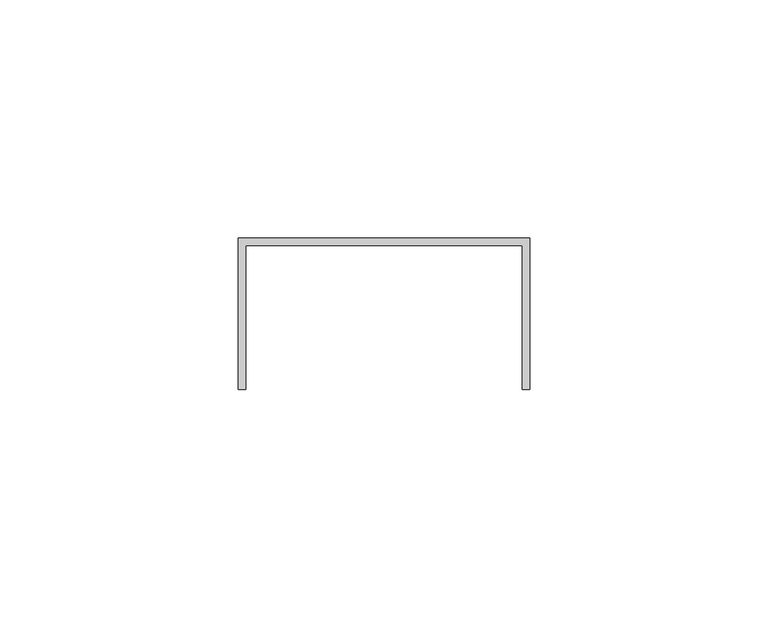
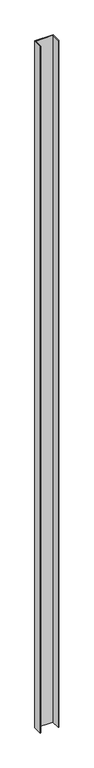
"""IFC4 building model written with IfcOpenShell, lengths in millimetres: proxy geometry, Generic Models 7:Generic Models 1:3:Generic Models 1:3 : Generic Models 7:Generic Models 1:305549:3:Generic Models 1:3:Generic Models 1:3 : Generic Models 7:Generic Models 1:305549:3 : Generic Models 7:Generic Models 1:3:Generic Models 1:3 : Generic Models 7:Generic Models 1:305549:301244:29 : Generic Models 7:Generic Models 1:3:Generic Models 1:3 : Generic Models 7:Generic Models 1:305549:3:Generic Models 1:3:Generic Models 1:3 : Generic Models 7:Generic Models 1:305549:3 : Generic Models 7:Generic Models 1:3:Generic Models 1:3 : Generic Models 7:Generic Models 1:305549:301244:308848."""

from ifc_helpers import new_model, si_unit, frame, origin, place, context, project, spatial, polyline, outline, extrude, source, transform, mapped, element, save


def generic_models_d2488738(model_context):
    return source(origin(), model_context, "Body", "SweptSolid", [
        extrude(outline(polyline([(579322.7929739, -578737.1663841), (579383.9117239, -578737.1663841), (579383.9117239, -578768.9163841), (579382.3242239, -578768.9163841), (579382.3242239, -578738.7538841), (579324.3804739, -578738.7538841), (579324.3804739, -578768.9163841), (579322.7929739, -578768.9163841), (579322.7929739, -578737.1663841)])), frame((0.0, 0.0, 3721.1), z_axis=(0.0, 0.0, 1.0), x_axis=(1.0, 0.0, 0.0)), (0.0, 0.0, 1.0), 2430.9324376),
    ])


if __name__ == "__main__":
    model = new_model("IFC4")
    model_context = context("Model", 3, world=origin())
    ifc_project = project(units=[si_unit("LENGTHUNIT", "METRE", prefix="MILLI")], contexts=[model_context])
    site = spatial("IfcSite", under=ifc_project)
    building = spatial("IfcBuilding", under=site)
    placement = place(None, origin())
    generic_models_shape = generic_models_d2488738(model_context)
    element("IfcBuildingElementProxy", 1, Name="Generic Models 7:Generic Models 1:3:Generic Models 1:3 : Generic Models 7:Generic Models 1:305549:3:Generic Models 1:3:Generic Models 1:3 : Generic Models 7:Generic Models 1:305549:3 : Generic Models 7:Generic Models 1:3:Generic Models 1:3 : Generic Models 7:Generic Models 1:305549:301244:29 : Generic Models 7:Generic Models 1:3:Generic Models 1:3 : Generic Models 7:Generic Models 1:305549:3:Generic Models 1:3:Generic Models 1:3 : Generic Models 7:Generic Models 1:305549:3 : Generic Models 7:Generic Models 1:3:Generic Models 1:3 : Generic Models 7:Generic Models 1:305549:301244:308848", ObjectType="Generic Models 7:Generic Models 1:3:Generic Models 1:3 : Generic Models 7:Generic Models 1:305549:3:Generic Models 1:3:Generic Models 1:3 : Generic Models 7:Generic Models 1:305549:3 : Generic Models 7:Generic Models 1:3:Generic Models 1:3 : Generic Models 7:Generic Models 1:305549:301244:29 : Generic Models 7:Generic Models 1:3:Generic Models 1:3 : Generic Models 7:Generic Models 1:305549:3:Generic Models 1:3:Generic Models 1:3 : Generic Models 7:Generic Models 1:305549:3 : Generic Models 7:Generic Models 1:3:Generic Models 1:3 : Generic Models 7:Generic Models 1:305549:301244:308848", at=placement, inside=building, context=model_context, shape_type="MappedRepresentation", body=[
        mapped(generic_models_shape, transform((0.0, 0.0, 0.0), x_axis=(1.0, 0.0, 0.0), y_axis=(0.0, 1.0, 0.0), z_axis=(0.0, 0.0, 1.0))),
    ])
    save(model, "model.ifc")

# Revit data of these elements
# Type "Generic Models 7:Generic Models 1:3:Generic Models 1:3 : Generic Models 7:Generic Models 1:305549:3:Generic Models 1:3:Generic Models 1:3 : Generic Models 7:Generic Models 1:305549:3 : Generic Models 7:Generic Models 1:3:Generic Models 1:3 : Generic Models 7:Generic Models 1:305549:301244:29 : Generic Models 7:Generic Models 1:3:Generic Models 1:3 : Generic Models 7:Generic Models 1:305549:3:Generic Models 1:3:Generic Models 1:3 : Generic Models 7:Generic Models 1:305549:3 : Generic Models 7:Generic Models 1:3:Generic Models 1:3 : Generic Models 7:Generic Models 1:305549:301244:308848"
#   NameOverride = "Generic Models 7:Generic Models 1:3:Generic Models 1:3 : Generic Models 7:Generic Models 1:305549:3:Generic Models 1:3:Generic Models 1:3 : Generic Models 7:Generic Models 1:305549:3 : Generic Models 7:Generic Models 1:3:Generic Models 1:3 : Generic Models 7:Generic Models 1:305549:301244:308848"
#   ObjectTypeOverride = "Generic Models 1:3:Generic Models 1:3 : Generic Models 7:Generic Models 1:305549:3 : Generic Models 7:Generic Models 1:3:Generic Models 1:3 : Generic Models 7:Generic Models 1:305549:301244"
#   Reference = "Generic Models 1"
#   Tag = "308848"
# Element 1 (IfcBuildingElementProxy, "Generic Models 7:Generic Models 1:3:Generic Models 1:3 : Generic Models 7:Generic Models 1:305549:3:Generic Models 1:3:Generic Models 1:3 : Generic Models 7:Generic Models 1:305549:3 : Generic Models 7:Generic Models 1:3:Generic Models 1:3 : Generic Models 7:Generic Models 1:305549:301244:29 : Generic Models 7:Generic Models 1:3:Generic Models 1:3 : Generic Models 7:Generic Models 1:305549:3:Generic Models 1:3:Generic Models 1:3 : Generic Models 7:Generic Models 1:305549:3 : Generic Models 7:Generic Models 1:3:Generic Models 1:3 : Generic Models 7:Generic Models 1:305549:301244:308848")
#   Materials on its faces: "GALVANIZED U-CHANNEL (250T125-33)"
# Materials
#   "GALVANIZED U-CHANNEL (250T125-33)": class "Unassigned", colour RGB 202 201 200, transparency 0, Keynote = "M05451300.02", Cost = 0
